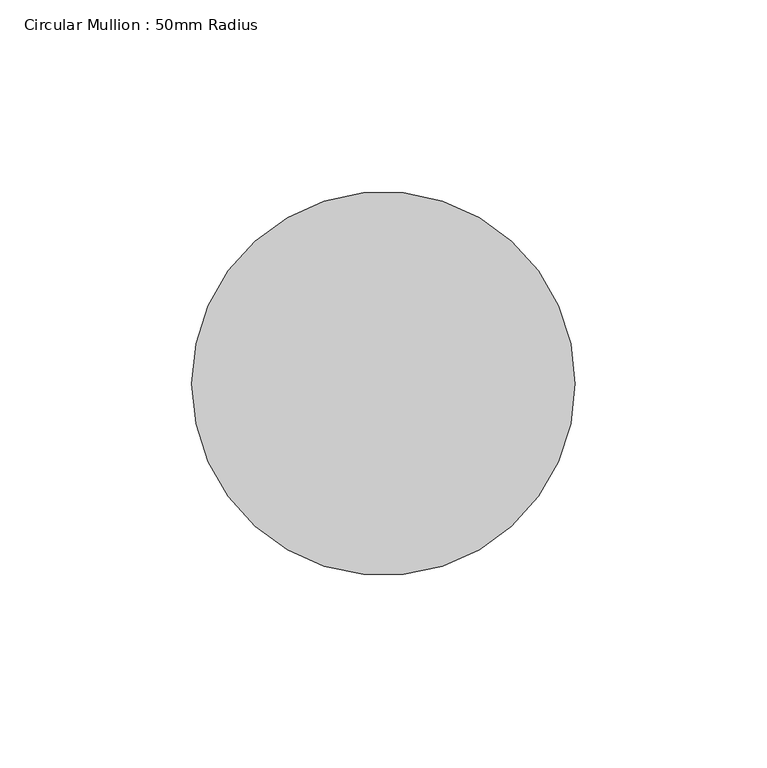
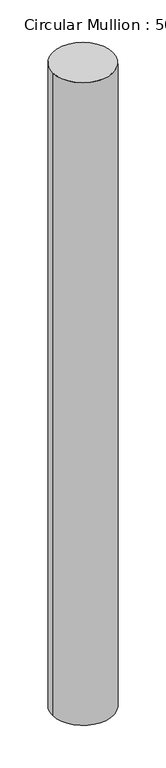
"""IFC4 building model written with IfcOpenShell, lengths in millimetres: member geometry, Circular Mullion : 50mm Radius."""

from ifc_helpers import new_model, si_unit, point, frame, origin, origin_2d, place, context, project, spatial, circle_curve, trimmed, segment, composite_curve, outline, extrude, source, transform, mapped, element, save


def circular_mullion_50mm_radius_2b4e5678(model_context):
    return source(origin(), model_context, "Body", "SweptSolid", [
        extrude(outline(composite_curve([segment(trimmed(circle_curve(origin_2d(), 50.0), [point((50.0, 0.0))], [point((-50.0, 0.0))], False, "CARTESIAN"), True, "CONTINUOUS"), segment(trimmed(circle_curve(origin_2d(), 50.0), [point((-50.0, 0.0))], [point((50.0, 0.0))], False, "CARTESIAN"), True, "CONTINUOUS")], self_intersect=False)), frame((0.0, 0.0, -1118.1190592), z_axis=(0.0, 0.0, 1.0), x_axis=(1.0, 0.0, 0.0)), (0.0, 0.0, 1.0), 1118.1190592),
    ])


if __name__ == "__main__":
    model = new_model("IFC4")
    model_context = context("Model", 3, world=origin())
    ifc_project = project(units=[si_unit("LENGTHUNIT", "METRE", prefix="MILLI")], contexts=[model_context])
    site = spatial("IfcSite", under=ifc_project)
    building = spatial("IfcBuilding", under=site)
    placement = place(None, origin())
    circular_mullion_50mm_radius_shape = circular_mullion_50mm_radius_2b4e5678(model_context)
    element("IfcMember", 1, ObjectType="Circular Mullion : 50mm Radius", at=placement, inside=building, context=model_context, shape_type="MappedRepresentation", body=[
        mapped(circular_mullion_50mm_radius_shape, transform((0.0, 0.0, 0.0), x_axis=(1.0, 0.0, 0.0), y_axis=(0.0, 1.0, 0.0), z_axis=(0.0, 0.0, 1.0))),
    ])
    save(model, "model.ifc")

# Revit data of these elements
# Type "Circular Mullion : 50mm Radius"
#   built-in parameter 1007350 = 0.164042 (stored number, unit not read)
# Element 1 (IfcMember, "Circular Mullion : 50mm Radius")
#   Materials on its faces: "Aluminium"
# Materials
#   "Aluminium": class "Metal", colour RGB 247 247 247, transparency 0, Description = "Aluminium 6061", Cost = 0
